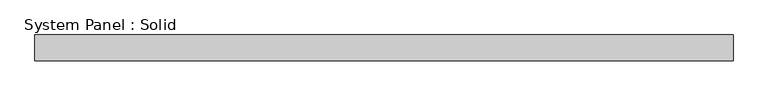
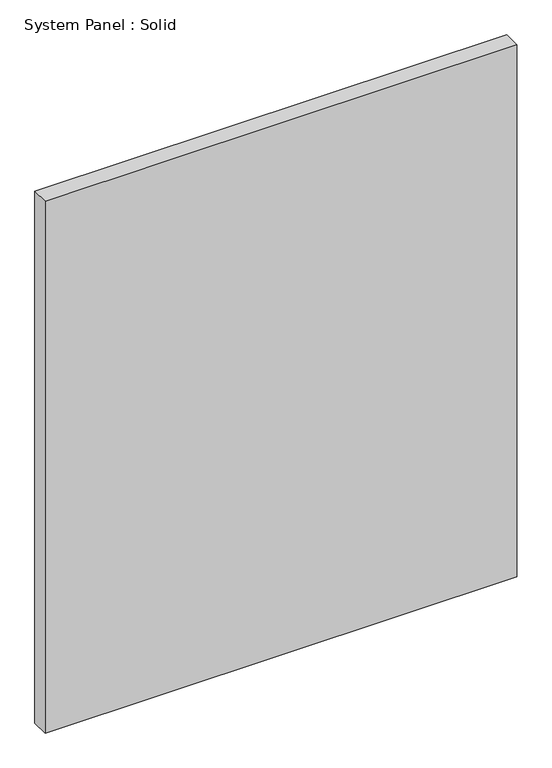
"""IFC4 building model written with IfcOpenShell, lengths in millimetres: plate geometry, System Panel : Solid."""

from ifc_helpers import new_model, si_unit, origin, origin_with_axes, place, context, project, spatial, polyline, outline, extrude, source, transform, mapped, element, save


def system_panel_solid_f77b040a(model_context):
    return source(origin(), model_context, "Body", "SweptSolid", [
        extrude(outline(polyline([(807.5, -10.5), (-807.5, -10.5), (-807.5, 49.5), (807.5, 49.5), (807.5, -10.5)])), origin_with_axes(), (0.0, 0.0, 1.0), 1925.0),
    ])


if __name__ == "__main__":
    model = new_model("IFC4")
    model_context = context("Model", 3, world=origin())
    ifc_project = project(units=[si_unit("LENGTHUNIT", "METRE", prefix="MILLI")], contexts=[model_context])
    site = spatial("IfcSite", under=ifc_project)
    building = spatial("IfcBuilding", under=site)
    placement = place(None, origin())
    system_panel_solid_shape = system_panel_solid_f77b040a(model_context)
    element("IfcPlate", 1, ObjectType="System Panel : Solid", at=placement, inside=building, context=model_context, shape_type="MappedRepresentation", body=[
        mapped(system_panel_solid_shape, transform((0.0, 0.0, 0.0), x_axis=(1.0, 0.0, 0.0), y_axis=(0.0, 1.0, 0.0), z_axis=(0.0, 0.0, 1.0))),
    ])
    save(model, "model.ifc")

# Revit data of these elements
# Element 1 (IfcPlate, "System Panel : Solid")
#   Materials on its faces: "Default"
# Materials
#   "Default": class "Miscellaneous", colour RGB 127 127 127, transparency 0
